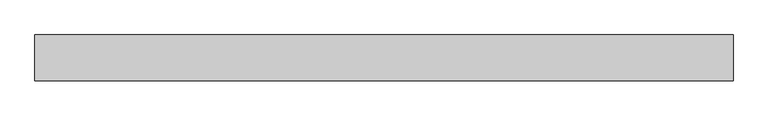
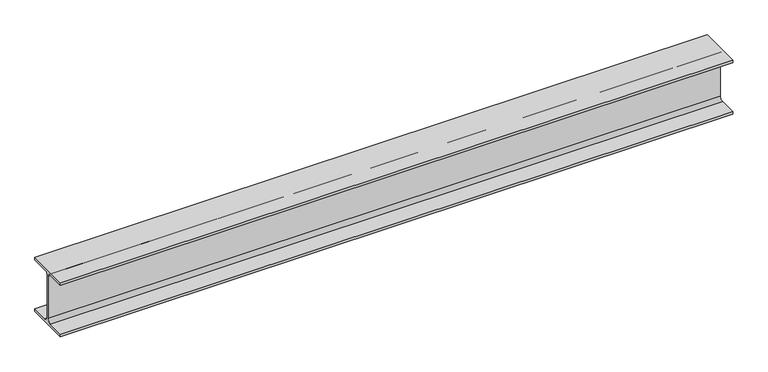
"""IFC4 building model written with IfcOpenShell, lengths in millimetres: beam geometry, 0912_Steel Framing_H-KSD3502 : H_SB_ASB_H-194x150x6x9."""

import ifcopenshell
import ifcopenshell.guid

model = None  # the IFC model being written
_history = None  # IfcOwnerHistory: only IFC2X3 demands one
_inside = {}  # id of a spatial element -> (the spatial element, [elements in it])
_under = {}  # id of a project, library or spatial element -> (it, [spatial elements below it])
_declared = {}  # id of a project -> (the project, [libraries it declares])
_typed = {}  # id of a type object -> (the type object, [elements of that type])
_made_of = {}  # id of a material, layer set ... -> (it, [elements and type objects made of it])


def new_model(schema):
    """Start an empty IFC model of exactly this schema.

    Asked for "IFC4X3", IfcOpenShell would pick the latest addendum, in which some entities
    have other attributes; the version numbers below select the first issue.
    IFC2X3 requires an IfcOwnerHistory on every rooted entity: one is made here for all.
    """
    global model, _history
    if schema == "IFC4X3":
        model = ifcopenshell.file(schema_version=(4, 3, 0, 0))
    else:
        model = ifcopenshell.file(schema=schema)
    _inside.clear()
    _under.clear()
    _declared.clear()
    _typed.clear()
    _made_of.clear()
    _history = None
    if model.schema == "IFC2X3":
        org = make("IfcOrganization", Name="unknown")
        user = make(
            "IfcPersonAndOrganization",
            ThePerson=make("IfcPerson", FamilyName="unknown"),
            TheOrganization=org,
        )
        app = make(
            "IfcApplication",
            ApplicationDeveloper=org,
            Version="unknown",
            ApplicationFullName="unknown",
            ApplicationIdentifier="unknown",
        )
        _history = make(
            "IfcOwnerHistory",
            OwningUser=user,
            OwningApplication=app,
            ChangeAction="ADDED",
            CreationDate=0,
        )
    return model


def make(cls, **values):
    """One entity of the class cls with the attributes given. An attribute that is None is left unset."""
    return model.create_entity(
        cls, **{name: value for name, value in values.items() if value is not None}
    )


def rooted(cls, **values):
    """An entity with a GlobalId (a new one), such as an element, a storey or a relation."""
    return make(cls, GlobalId=ifcopenshell.guid.new(), OwnerHistory=_history, **values)


def si_unit(unit_type, name, prefix=None):
    """IfcSIUnit, for example si_unit("LENGTHUNIT", "METRE", prefix="MILLI")."""
    return make("IfcSIUnit", UnitType=unit_type, Prefix=prefix, Name=name)


def assignment(units):
    """IfcUnitAssignment: the units of a project."""
    return None if units is None else make("IfcUnitAssignment", Units=units)


def point(xyz):
    """IfcCartesianPoint."""
    return None if xyz is None else make("IfcCartesianPoint", Coordinates=xyz)


def direction(xyz):
    """IfcDirection."""
    return None if xyz is None else make("IfcDirection", DirectionRatios=xyz)


def frame(location, z_axis=None, x_axis=None):
    """IfcAxis2Placement3D, a coordinate frame: its origin and axes. An axis left out is left unset."""
    return make(
        "IfcAxis2Placement3D",
        Location=point(location),
        Axis=direction(z_axis),
        RefDirection=direction(x_axis),
    )


def frame_2d(location, x_axis=None):
    """IfcAxis2Placement2D, a coordinate frame in the plane: its origin and x axis."""
    return make(
        "IfcAxis2Placement2D", Location=point(location), RefDirection=direction(x_axis)
    )


def origin():
    """The frame at (0, 0, 0) with its axes left unset."""
    return frame((0.0, 0.0, 0.0))


def place(relative_to, where):
    """IfcLocalPlacement: puts the frame where relative to a parent placement (None: the world)."""
    return make(
        "IfcLocalPlacement", PlacementRelTo=relative_to, RelativePlacement=where
    )


def context(
    kind, dimensions, precision=None, world=None, true_north=None, identifier=None
):
    """IfcGeometricRepresentationContext, for example the 3D "Model" context."""
    return make(
        "IfcGeometricRepresentationContext",
        ContextIdentifier=identifier,
        ContextType=kind,
        CoordinateSpaceDimension=dimensions,
        Precision=precision,
        WorldCoordinateSystem=world,
        TrueNorth=true_north,
    )


def project(units=None, contexts=None):
    """IfcProject with its units and contexts."""
    return rooted(
        "IfcProject",
        Name="project",
        RepresentationContexts=contexts,
        UnitsInContext=assignment(units),
    )


def spatial(cls, under=None, at=None, **own):
    """A site, building, storey or space (cls), placed at a placement, below another one or the project."""
    s = rooted(cls, ObjectPlacement=at, **own)
    if under is not None:
        _under.setdefault(under.id(), (under, []))[1].append(s)
    return s


def polyline(points):
    """IfcPolyline through the points."""
    return make("IfcPolyline", Points=[point(p) for p in points])


def circle_curve(where, radius):
    """IfcCircle in the frame where."""
    return make("IfcCircle", Position=where, Radius=radius)


def trimmed(basis, trim1, trim2, sense, master):
    """IfcTrimmedCurve: the piece of a basis curve between two trims."""
    return make(
        "IfcTrimmedCurve",
        BasisCurve=basis,
        Trim1=trim1,
        Trim2=trim2,
        SenseAgreement=sense,
        MasterRepresentation=master,
    )


def segment(curve, same_sense, transition):
    """IfcCompositeCurveSegment."""
    return make(
        "IfcCompositeCurveSegment",
        Transition=transition,
        SameSense=same_sense,
        ParentCurve=curve,
    )


def composite_curve(segments, self_intersect=None):
    """IfcCompositeCurve: segments joined end to end."""
    return make("IfcCompositeCurve", Segments=segments, SelfIntersect=self_intersect)


def outline(outer, holes=None, kind="AREA"):
    """IfcArbitraryClosedProfileDef: a profile drawn as a closed curve; with holes, ...WithVoids."""
    if holes is None:
        return make("IfcArbitraryClosedProfileDef", ProfileType=kind, OuterCurve=outer)
    return make(
        "IfcArbitraryProfileDefWithVoids",
        ProfileType=kind,
        OuterCurve=outer,
        InnerCurves=holes,
    )


def extrude(swept, where, along, depth):
    """IfcExtrudedAreaSolid: the profile swept, set in the frame where, extruded along a direction by depth."""
    return make(
        "IfcExtrudedAreaSolid",
        SweptArea=swept,
        Position=where,
        ExtrudedDirection=direction(along),
        Depth=depth,
    )


def shape(context_of_items, identifier, shape_type, items):
    """IfcShapeRepresentation: the items that make up one representation, for example the "Body"."""
    return make(
        "IfcShapeRepresentation",
        ContextOfItems=context_of_items,
        RepresentationIdentifier=identifier,
        RepresentationType=shape_type,
        Items=items,
    )


def source(mapping_origin, context_of_items, identifier, shape_type, items):
    """IfcRepresentationMap: a shape defined once, which mapped items show again and again."""
    return make(
        "IfcRepresentationMap",
        MappingOrigin=mapping_origin,
        MappedRepresentation=shape(context_of_items, identifier, shape_type, items),
    )


def transform(
    local_origin,
    x_axis=None,
    y_axis=None,
    z_axis=None,
    scale=None,
    scale2=None,
    scale3=None,
    uniform=True,
):
    """IfcCartesianTransformationOperator3D, or its non-uniform kind. x_axis, y_axis, z_axis: its Axis1, 2, 3."""
    if uniform:
        return make(
            "IfcCartesianTransformationOperator3D",
            Axis1=direction(x_axis),
            Axis2=direction(y_axis),
            LocalOrigin=point(local_origin),
            Scale=scale,
            Axis3=direction(z_axis),
        )
    return make(
        "IfcCartesianTransformationOperator3DnonUniform",
        Axis1=direction(x_axis),
        Axis2=direction(y_axis),
        LocalOrigin=point(local_origin),
        Scale=scale,
        Axis3=direction(z_axis),
        Scale2=scale2,
        Scale3=scale3,
    )


def mapped(mapping_source, mapping_target):
    """IfcMappedItem: shows the shape of a source again, moved by a transform."""
    return make(
        "IfcMappedItem", MappingSource=mapping_source, MappingTarget=mapping_target
    )


def made_of(thing, what):
    """Note that an element or type object is made of a material, layer set ...; save() writes the relation."""
    if what is not None:
        _made_of.setdefault(what.id(), (what, []))[1].append(thing)
    return thing


def element(
    cls,
    number,
    at=None,
    inside=None,
    cuts=None,
    type_object=None,
    material=None,
    context=None,
    identifier="Body",
    shape_type=None,
    held_by="IfcProductDefinitionShape",
    body=None,
    shapes=None,
    **own,
):
    """One element of the class cls, such as IfcWall. Its Tag is "e" and its number.

    at: its placement. inside: the storey or other place that contains it. cuts: it is an
    opening in that element (IfcRelVoidsElement). A single representation is given by context,
    identifier, shape_type and body (its items); several are given by shapes. held_by: the class
    of the entity that holds the representations. save() writes the other relations.
    """
    e = rooted(cls, Tag="e%d" % number, ObjectPlacement=at, **own)
    if body is not None:
        shapes = [shape(context, identifier, shape_type, body)]
    if shapes is not None:
        e.Representation = make(held_by, Representations=shapes)
    if inside is not None:
        _inside.setdefault(inside.id(), (inside, []))[1].append(e)
    if cuts is not None:
        rooted(
            "IfcRelVoidsElement", RelatingBuildingElement=cuts, RelatedOpeningElement=e
        )
    if type_object is not None:
        _typed.setdefault(type_object.id(), (type_object, []))[1].append(e)
    return made_of(e, material)


def aggregate(whole, parts):
    """IfcRelAggregates: a whole, such as a stair, and the parts it consists of."""
    return rooted("IfcRelAggregates", RelatingObject=whole, RelatedObjects=parts)


def save(model, path):
    """Write the relations noted so far, then the file.

    IfcRelAggregates (storeys below a building ...), IfcRelContainedInSpatialStructure (elements
    in a storey), IfcRelDefinesByType, IfcRelAssociatesMaterial and IfcRelDeclares: one each for
    every whole, place, type object, material and project.
    """
    for whole, parts in _under.values():
        aggregate(whole, parts)
    for where, things in _inside.values():
        rooted(
            "IfcRelContainedInSpatialStructure",
            RelatedElements=things,
            RelatingStructure=where,
        )
    for kind, things in _typed.values():
        rooted("IfcRelDefinesByType", RelatedObjects=things, RelatingType=kind)
    for what, things in _made_of.values():
        rooted("IfcRelAssociatesMaterial", RelatedObjects=things, RelatingMaterial=what)
    for by, libraries in _declared.values():
        rooted("IfcRelDeclares", RelatingContext=by, RelatedDefinitions=libraries)
    model.write(path)


def beam_a62f083a(model_context):
    return source(origin(), model_context, "Body", "SweptSolid", [
        extrude(outline(composite_curve([segment(polyline([(-75.0, -88.0), (-16.0, -88.0)]), True, "CONTINUOUS"), segment(trimmed(circle_curve(frame_2d((-16.0, -75.0)), 13.0), [point((-16.0, -88.0))], [point((-3.0, -75.0))], True, "CARTESIAN"), True, "CONTINUOUS"), segment(polyline([(-3.0, -75.0), (-3.0, 75.0)]), True, "CONTINUOUS"), segment(trimmed(circle_curve(frame_2d((-16.0, 75.0)), 13.0), [point((-3.0, 75.0))], [point((-16.0, 88.0))], True, "CARTESIAN"), True, "CONTINUOUS"), segment(polyline([(-16.0, 88.0), (-75.0, 88.0), (-75.0, 97.0), (75.0, 97.0), (75.0, 88.0), (16.0, 88.0)]), True, "CONTINUOUS"), segment(trimmed(circle_curve(frame_2d((16.0, 75.0)), 13.0), [point((16.0, 88.0))], [point((3.0, 75.0))], True, "CARTESIAN"), True, "CONTINUOUS"), segment(polyline([(3.0, 75.0), (3.0, -75.0)]), True, "CONTINUOUS"), segment(trimmed(circle_curve(frame_2d((16.0, -75.0)), 13.0), [point((3.0, -75.0))], [point((16.0, -88.0))], True, "CARTESIAN"), True, "CONTINUOUS"), segment(polyline([(16.0, -88.0), (75.0, -88.0), (75.0, -97.0), (-75.0, -97.0), (-75.0, -88.0)]), True, "CONTINUOUS")], self_intersect=False)), frame((-700.4863388, 0.0, 0.0), z_axis=(1.0, 0.0, 0.0), x_axis=(0.0, 1.0, 0.0)), (0.0, 0.0, 1.0), 2280.3480504),
    ])


if __name__ == "__main__":
    model = new_model("IFC4")
    model_context = context("Model", 3, world=origin())
    ifc_project = project(units=[si_unit("LENGTHUNIT", "METRE", prefix="MILLI")], contexts=[model_context])
    site = spatial("IfcSite", under=ifc_project)
    building = spatial("IfcBuilding", under=site)
    placement = place(None, origin())
    beam_shape = beam_a62f083a(model_context)
    element("IfcBeam", 1, ObjectType="0912_Steel Framing_H-KSD3502 : H_SB_ASB_H-194x150x6x9", at=placement, inside=building, context=model_context, shape_type="MappedRepresentation", body=[
        mapped(beam_shape, transform((0.0, 0.0, 0.0), x_axis=(1.0, 0.0, 0.0), y_axis=(0.0, 1.0, 0.0), z_axis=(0.0, 0.0, 1.0))),
    ])
    save(model, "model.ifc")

# Revit data of these elements
# Type "0912_Steel Framing_H-KSD3502 : H_SB_ASB_H-194x150x6x9"
#   H_WM Code_1 = "S01AA002-00001 | Main Steel Structure Fabrication Work | Shelter/Building | Medium Steel - Standard (90KG/M>Weight≥30KG/M) | Material: (   )"
#   H_WM Code_2 = "S03AA028-00001 | Main Steel Structure Erection Work | Shelter/Building | Medium Steel (90KG/M>Weight≥30KG/M) | Material: (   )"
#   H_WM Code_3 = "S01AA010-00001 | Main Steel Structure Fabrication Work | Shelter/Building | Steel Painting/Coating | for Non-Fireproofed Steel Surface, Surface Preparation, Primer, Second & Final Coat | Material: (   )"
#   H_Q'ty Cal Type Tag = "SB-Q2"
#   Width = 15.0 cm
#   Web Thickness = 0.6 cm
#   Web Fillet = 1.3 cm
#   Warping Constant = 43316.0 cm⁶
#   W = 0
#   Torsional Moment of Inertia = 8.622 cm⁴
#   Section Area = 39.01 cm²
#   Plastic Modulus weak axis = 104.0 cm³
#   Plastic Modulus strong axis = 309.0 cm³
#   Perimeter = 0.95 m²/m
#   Nominal Weight = 30.60 kgf/m
#   Moment of Inertia weak axis = 507.00 cm⁴
#   Moment of Inertia strong axis = 2690.00 cm⁴
#   Height = 19.4 cm
#   Flange Thickness = 0.9 cm
#   Elastic Modulus weak axis = 67.6 cm³
#   Elastic Modulus strong axis = 277.0 cm³
#   Centroid Vertical = 9.7 cm
#   Centroid Horizontal = 7.5 cm
#   Ix = 26900000
#   Length [instance default] = 1.5240 m
#   Zx = 309000
#   b = 0.1500 m
#   h = 0.1940 m
#   r = 0.0130 m
#   s = 0.0060 m
#   t = 0.0090 m
#   A = 0.003901 m²
#   Structural Material [instance default] = Steel, 45-345
#   Assembly Code = ""
# Element 1 (IfcBeam, "0912_Steel Framing_H-KSD3502 : H_SB_ASB_H-194x150x6x9")
#   Structural Material = none
# Materials
#   "Steel, 45-345": class "Metal", colour RGB 189 187 185, transparency 0, Description = "Steel 345 MPa", Cost = 0
